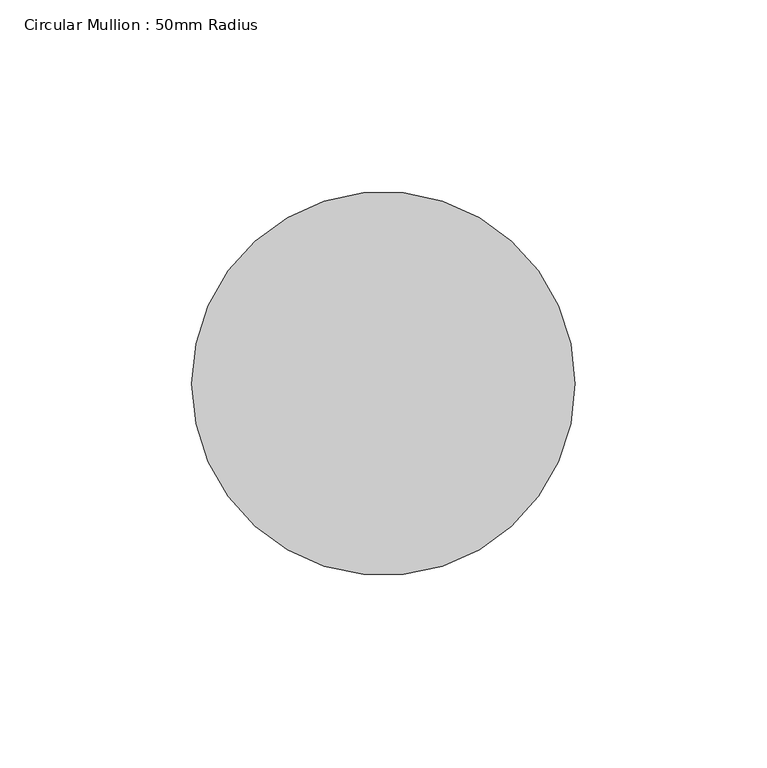
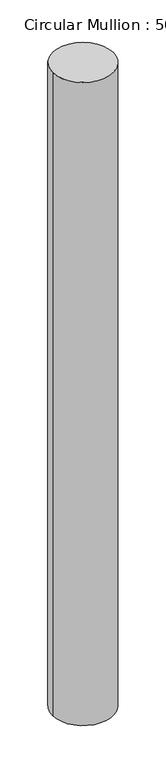
"""IFC4 building model written with IfcOpenShell, lengths in millimetres: member geometry, Circular Mullion : 50mm Radius."""

from ifc_helpers import new_model, si_unit, point, frame, origin, origin_2d, place, context, project, spatial, circle_curve, trimmed, segment, composite_curve, outline, extrude, source, transform, mapped, element, save


def circular_mullion_50mm_radius_de7e4bc6(model_context):
    return source(origin(), model_context, "Body", "SweptSolid", [
        extrude(outline(composite_curve([segment(trimmed(circle_curve(origin_2d(), 50.0), [point((50.0, 0.0))], [point((-50.0, 0.0))], False, "CARTESIAN"), True, "CONTINUOUS"), segment(trimmed(circle_curve(origin_2d(), 50.0), [point((-50.0, 0.0))], [point((50.0, 0.0))], False, "CARTESIAN"), True, "CONTINUOUS")], self_intersect=False)), frame((0.0, 0.0, -1121.2246738), z_axis=(0.0, 0.0, 1.0), x_axis=(1.0, 0.0, 0.0)), (0.0, 0.0, 1.0), 1121.2246738),
    ])


if __name__ == "__main__":
    model = new_model("IFC4")
    model_context = context("Model", 3, world=origin())
    ifc_project = project(units=[si_unit("LENGTHUNIT", "METRE", prefix="MILLI")], contexts=[model_context])
    site = spatial("IfcSite", under=ifc_project)
    building = spatial("IfcBuilding", under=site)
    placement = place(None, origin())
    circular_mullion_50mm_radius_shape = circular_mullion_50mm_radius_de7e4bc6(model_context)
    element("IfcMember", 1, ObjectType="Circular Mullion : 50mm Radius", at=placement, inside=building, context=model_context, shape_type="MappedRepresentation", body=[
        mapped(circular_mullion_50mm_radius_shape, transform((0.0, 0.0, 0.0), x_axis=(1.0, 0.0, 0.0), y_axis=(0.0, 1.0, 0.0), z_axis=(0.0, 0.0, 1.0))),
    ])
    save(model, "model.ifc")

# Revit data of these elements
# Type "Circular Mullion : 50mm Radius"
#   built-in parameter 1007350 = 0.164042 (stored number, unit not read)
# Element 1 (IfcMember, "Circular Mullion : 50mm Radius")
#   Materials on its faces: "Aluminium"
# Materials
#   "Aluminium": class "Metal", colour RGB 247 247 247, transparency 0, Description = "Aluminium 6061", Cost = 0
